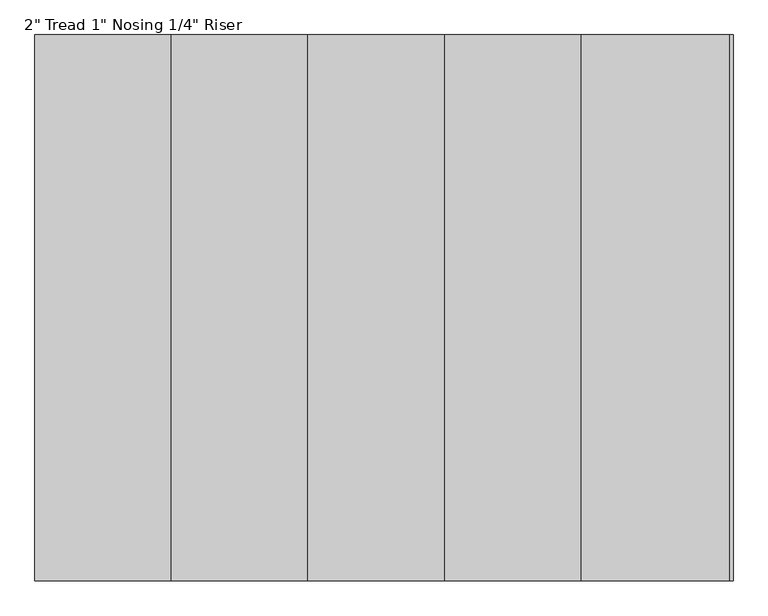
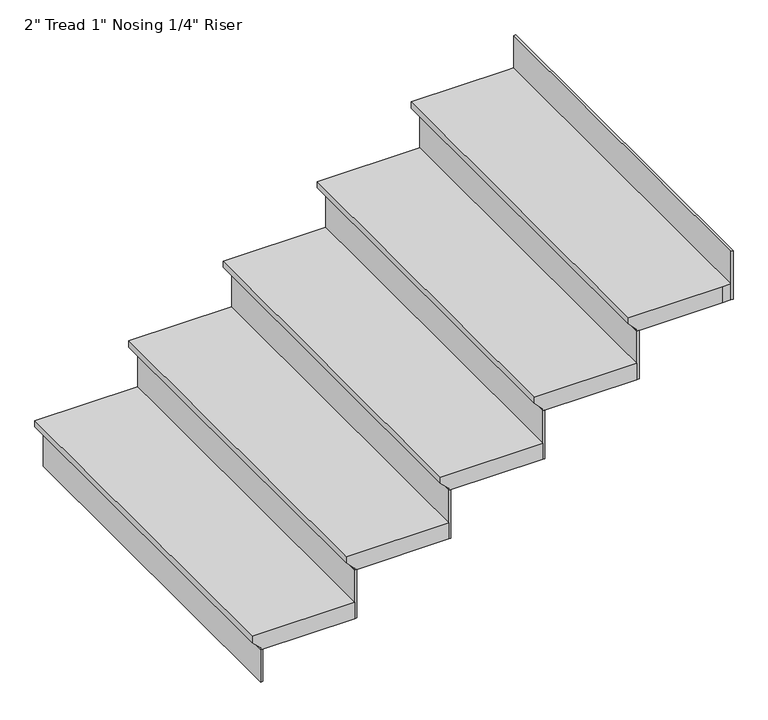
"""IFC4 building model written with IfcOpenShell, lengths in millimetres: stair flight geometry."""

import ifcopenshell
import ifcopenshell.guid

model = None  # the IFC model being written
_history = None  # IfcOwnerHistory: only IFC2X3 demands one
_inside = {}  # id of a spatial element -> (the spatial element, [elements in it])
_under = {}  # id of a project, library or spatial element -> (it, [spatial elements below it])
_declared = {}  # id of a project -> (the project, [libraries it declares])
_typed = {}  # id of a type object -> (the type object, [elements of that type])
_made_of = {}  # id of a material, layer set ... -> (it, [elements and type objects made of it])


def new_model(schema):
    """Start an empty IFC model of exactly this schema.

    Asked for "IFC4X3", IfcOpenShell would pick the latest addendum, in which some entities
    have other attributes; the version numbers below select the first issue.
    IFC2X3 requires an IfcOwnerHistory on every rooted entity: one is made here for all.
    """
    global model, _history
    if schema == "IFC4X3":
        model = ifcopenshell.file(schema_version=(4, 3, 0, 0))
    else:
        model = ifcopenshell.file(schema=schema)
    _inside.clear()
    _under.clear()
    _declared.clear()
    _typed.clear()
    _made_of.clear()
    _history = None
    if model.schema == "IFC2X3":
        org = make("IfcOrganization", Name="unknown")
        user = make(
            "IfcPersonAndOrganization",
            ThePerson=make("IfcPerson", FamilyName="unknown"),
            TheOrganization=org,
        )
        app = make(
            "IfcApplication",
            ApplicationDeveloper=org,
            Version="unknown",
            ApplicationFullName="unknown",
            ApplicationIdentifier="unknown",
        )
        _history = make(
            "IfcOwnerHistory",
            OwningUser=user,
            OwningApplication=app,
            ChangeAction="ADDED",
            CreationDate=0,
        )
    return model


def make(cls, **values):
    """One entity of the class cls with the attributes given. An attribute that is None is left unset."""
    return model.create_entity(
        cls, **{name: value for name, value in values.items() if value is not None}
    )


def rooted(cls, **values):
    """An entity with a GlobalId (a new one), such as an element, a storey or a relation."""
    return make(cls, GlobalId=ifcopenshell.guid.new(), OwnerHistory=_history, **values)


def si_unit(unit_type, name, prefix=None):
    """IfcSIUnit, for example si_unit("LENGTHUNIT", "METRE", prefix="MILLI")."""
    return make("IfcSIUnit", UnitType=unit_type, Prefix=prefix, Name=name)


def assignment(units):
    """IfcUnitAssignment: the units of a project."""
    return None if units is None else make("IfcUnitAssignment", Units=units)


def point(xyz):
    """IfcCartesianPoint."""
    return None if xyz is None else make("IfcCartesianPoint", Coordinates=xyz)


def direction(xyz):
    """IfcDirection."""
    return None if xyz is None else make("IfcDirection", DirectionRatios=xyz)


def frame(location, z_axis=None, x_axis=None):
    """IfcAxis2Placement3D, a coordinate frame: its origin and axes. An axis left out is left unset."""
    return make(
        "IfcAxis2Placement3D",
        Location=point(location),
        Axis=direction(z_axis),
        RefDirection=direction(x_axis),
    )


def origin():
    """The frame at (0, 0, 0) with its axes left unset."""
    return frame((0.0, 0.0, 0.0))


def place(relative_to, where):
    """IfcLocalPlacement: puts the frame where relative to a parent placement (None: the world)."""
    return make(
        "IfcLocalPlacement", PlacementRelTo=relative_to, RelativePlacement=where
    )


def context(
    kind, dimensions, precision=None, world=None, true_north=None, identifier=None
):
    """IfcGeometricRepresentationContext, for example the 3D "Model" context."""
    return make(
        "IfcGeometricRepresentationContext",
        ContextIdentifier=identifier,
        ContextType=kind,
        CoordinateSpaceDimension=dimensions,
        Precision=precision,
        WorldCoordinateSystem=world,
        TrueNorth=true_north,
    )


def project(units=None, contexts=None):
    """IfcProject with its units and contexts."""
    return rooted(
        "IfcProject",
        Name="project",
        RepresentationContexts=contexts,
        UnitsInContext=assignment(units),
    )


def spatial(cls, under=None, at=None, **own):
    """A site, building, storey or space (cls), placed at a placement, below another one or the project."""
    s = rooted(cls, ObjectPlacement=at, **own)
    if under is not None:
        _under.setdefault(under.id(), (under, []))[1].append(s)
    return s


def faces_of(points, faces, orient=None, outer=None):
    """IfcFace entities. A face is a list of loops; a loop is a list of indices into points, from 0.

    orient and outer hold one flag for each loop. By default every Orientation is true, the
    first loop of a face is its IfcFaceOuterBound and the others are IfcFaceBound.
    """
    made = []
    for i, loops in enumerate(faces):
        bounds = []
        for j, loop in enumerate(loops):
            is_outer = j == 0 if outer is None else outer[i][j]
            bounds.append(
                make(
                    "IfcFaceOuterBound" if is_outer else "IfcFaceBound",
                    Bound=make("IfcPolyLoop", Polygon=[points[k] for k in loop]),
                    Orientation=True if orient is None else orient[i][j],
                )
            )
        made.append(make("IfcFace", Bounds=bounds))
    return made


def faceted_brep(points, faces, orient=None, outer=None, voids=None):
    """IfcFacetedBrep: a solid bounded by flat faces; with voids (closed shells), ...WithVoids."""
    shared = [point(p) for p in points]
    hull = make("IfcClosedShell", CfsFaces=faces_of(shared, faces, orient, outer))
    if voids is None:
        return make("IfcFacetedBrep", Outer=hull)
    return make(
        "IfcFacetedBrepWithVoids",
        Outer=hull,
        Voids=[
            make(cls, CfsFaces=faces_of(shared, fs, o, b)) for cls, fs, o, b in voids
        ],
    )


def shape(context_of_items, identifier, shape_type, items):
    """IfcShapeRepresentation: the items that make up one representation, for example the "Body"."""
    return make(
        "IfcShapeRepresentation",
        ContextOfItems=context_of_items,
        RepresentationIdentifier=identifier,
        RepresentationType=shape_type,
        Items=items,
    )


def source(mapping_origin, context_of_items, identifier, shape_type, items):
    """IfcRepresentationMap: a shape defined once, which mapped items show again and again."""
    return make(
        "IfcRepresentationMap",
        MappingOrigin=mapping_origin,
        MappedRepresentation=shape(context_of_items, identifier, shape_type, items),
    )


def transform(
    local_origin,
    x_axis=None,
    y_axis=None,
    z_axis=None,
    scale=None,
    scale2=None,
    scale3=None,
    uniform=True,
):
    """IfcCartesianTransformationOperator3D, or its non-uniform kind. x_axis, y_axis, z_axis: its Axis1, 2, 3."""
    if uniform:
        return make(
            "IfcCartesianTransformationOperator3D",
            Axis1=direction(x_axis),
            Axis2=direction(y_axis),
            LocalOrigin=point(local_origin),
            Scale=scale,
            Axis3=direction(z_axis),
        )
    return make(
        "IfcCartesianTransformationOperator3DnonUniform",
        Axis1=direction(x_axis),
        Axis2=direction(y_axis),
        LocalOrigin=point(local_origin),
        Scale=scale,
        Axis3=direction(z_axis),
        Scale2=scale2,
        Scale3=scale3,
    )


def mapped(mapping_source, mapping_target):
    """IfcMappedItem: shows the shape of a source again, moved by a transform."""
    return make(
        "IfcMappedItem", MappingSource=mapping_source, MappingTarget=mapping_target
    )


def made_of(thing, what):
    """Note that an element or type object is made of a material, layer set ...; save() writes the relation."""
    if what is not None:
        _made_of.setdefault(what.id(), (what, []))[1].append(thing)
    return thing


def element(
    cls,
    number,
    at=None,
    inside=None,
    cuts=None,
    type_object=None,
    material=None,
    context=None,
    identifier="Body",
    shape_type=None,
    held_by="IfcProductDefinitionShape",
    body=None,
    shapes=None,
    **own,
):
    """One element of the class cls, such as IfcWall. Its Tag is "e" and its number.

    at: its placement. inside: the storey or other place that contains it. cuts: it is an
    opening in that element (IfcRelVoidsElement). A single representation is given by context,
    identifier, shape_type and body (its items); several are given by shapes. held_by: the class
    of the entity that holds the representations. save() writes the other relations.
    """
    e = rooted(cls, Tag="e%d" % number, ObjectPlacement=at, **own)
    if body is not None:
        shapes = [shape(context, identifier, shape_type, body)]
    if shapes is not None:
        e.Representation = make(held_by, Representations=shapes)
    if inside is not None:
        _inside.setdefault(inside.id(), (inside, []))[1].append(e)
    if cuts is not None:
        rooted(
            "IfcRelVoidsElement", RelatingBuildingElement=cuts, RelatedOpeningElement=e
        )
    if type_object is not None:
        _typed.setdefault(type_object.id(), (type_object, []))[1].append(e)
    return made_of(e, material)


def aggregate(whole, parts):
    """IfcRelAggregates: a whole, such as a stair, and the parts it consists of."""
    return rooted("IfcRelAggregates", RelatingObject=whole, RelatedObjects=parts)


def save(model, path):
    """Write the relations noted so far, then the file.

    IfcRelAggregates (storeys below a building ...), IfcRelContainedInSpatialStructure (elements
    in a storey), IfcRelDefinesByType, IfcRelAssociatesMaterial and IfcRelDeclares: one each for
    every whole, place, type object, material and project.
    """
    for whole, parts in _under.values():
        aggregate(whole, parts)
    for where, things in _inside.values():
        rooted(
            "IfcRelContainedInSpatialStructure",
            RelatedElements=things,
            RelatingStructure=where,
        )
    for kind, things in _typed.values():
        rooted("IfcRelDefinesByType", RelatedObjects=things, RelatingType=kind)
    for what, things in _made_of.values():
        rooted("IfcRelAssociatesMaterial", RelatedObjects=things, RelatingMaterial=what)
    for by, libraries in _declared.values():
        rooted("IfcRelDeclares", RelatingContext=by, RelatedDefinitions=libraries)
    model.write(path)


def stair_flight_71736acc(model_context):
    return source(origin(), model_context, "Body", "Brep", [
        faceted_brep([(-2715.2122732, 8132.6265304, -781.05), (-2715.2122732, 8132.6265304, -762.0), (-2715.2122732, 9250.2265304, -762.0), (-2715.2122732, 9250.2265304, -781.05), (-2689.8122732, 8132.6265304, -806.45), (-2689.8122732, 9250.2265304, -806.45), (-2410.4122732, 8132.6265304, -762.0), (-2410.4122732, 9250.2265304, -762.0), (-2689.8122732, 9250.2265304, -812.8), (-2410.4122732, 9250.2265304, -812.8), (-2410.4122732, 8132.6265304, -812.8), (-2689.8122732, 8132.6265304, -812.8)], [[[0, 1, 2, 3]], [[4, 0, 3, 5]], [[2, 1, 6, 7]], [[8, 9, 10, 11]], [[2, 7, 9, 8, 5, 3]], [[8, 11, 4, 5]], [[6, 1, 0, 4, 11, 10]], [[7, 6, 10, 9]]]),
        faceted_brep([(-2689.8122732, 8132.6265304, -812.8), (-2689.8122732, 8132.6265304, -914.4), (-2683.4622732, 8132.6265304, -914.4), (-2683.4622732, 8132.6265304, -812.8), (-2689.8122732, 9250.2265304, -812.8), (-2683.4622732, 9250.2265304, -812.8), (-2683.4622732, 9250.2265304, -914.4), (-2689.8122732, 9250.2265304, -914.4)], [[[0, 1, 2, 3]], [[4, 5, 6, 7]], [[1, 0, 4, 7]], [[2, 1, 7, 6]], [[3, 2, 6, 5]], [[0, 3, 5, 4]]]),
        faceted_brep([(-2410.4122732, 8132.6265304, -660.4), (-2410.4122732, 8132.6265304, -812.8), (-2404.0622732, 8132.6265304, -812.8), (-2404.0622732, 8132.6265304, -660.4), (-2410.4122732, 9250.2265304, -660.4), (-2404.0622732, 9250.2265304, -660.4), (-2404.0622732, 9250.2265304, -812.8), (-2410.4122732, 9250.2265304, -812.8)], [[[0, 1, 2, 3]], [[4, 5, 6, 7]], [[1, 0, 4, 7]], [[2, 1, 7, 6]], [[3, 2, 6, 5]], [[0, 3, 5, 4]]]),
        faceted_brep([(-2435.8122732, 9250.2265304, -609.6), (-2435.8122732, 8132.6265304, -609.6), (-2131.0122732, 8132.6265304, -609.6), (-2131.0122732, 9250.2265304, -609.6), (-2410.4122732, 9250.2265304, -660.4), (-2131.0122732, 9250.2265304, -660.4), (-2131.0122732, 8132.6265304, -660.4), (-2410.4122732, 8132.6265304, -660.4), (-2410.4122732, 9250.2265304, -654.05), (-2435.8122732, 9250.2265304, -628.65), (-2410.4122732, 8132.6265304, -654.05), (-2435.8122732, 8132.6265304, -628.65)], [[[0, 1, 2, 3]], [[4, 5, 6, 7]], [[0, 3, 5, 4, 8, 9]], [[4, 7, 10, 8]], [[2, 1, 11, 10, 7, 6]], [[3, 2, 6, 5]], [[11, 1, 0, 9]], [[10, 11, 9, 8]]]),
        faceted_brep([(-2131.0122732, 8132.6265304, -508.0), (-2131.0122732, 8132.6265304, -660.4), (-2124.6622732, 8132.6265304, -660.4), (-2124.6622732, 8132.6265304, -508.0), (-2131.0122732, 9250.2265304, -508.0), (-2124.6622732, 9250.2265304, -508.0), (-2124.6622732, 9250.2265304, -660.4), (-2131.0122732, 9250.2265304, -660.4)], [[[0, 1, 2, 3]], [[4, 5, 6, 7]], [[1, 0, 4, 7]], [[2, 1, 7, 6]], [[3, 2, 6, 5]], [[0, 3, 5, 4]]]),
        faceted_brep([(-2156.4122732, 9250.2265304, -457.2), (-2156.4122732, 8132.6265304, -457.2), (-1851.6122732, 8132.6265304, -457.2), (-1851.6122732, 9250.2265304, -457.2), (-2131.0122732, 9250.2265304, -508.0), (-1851.6122732, 9250.2265304, -508.0), (-1851.6122732, 8132.6265304, -508.0), (-2131.0122732, 8132.6265304, -508.0), (-2131.0122732, 9250.2265304, -501.65), (-2156.4122732, 9250.2265304, -476.25), (-2131.0122732, 8132.6265304, -501.65), (-2156.4122732, 8132.6265304, -476.25)], [[[0, 1, 2, 3]], [[4, 5, 6, 7]], [[0, 3, 5, 4, 8, 9]], [[4, 7, 10, 8]], [[2, 1, 11, 10, 7, 6]], [[3, 2, 6, 5]], [[11, 1, 0, 9]], [[10, 11, 9, 8]]]),
        faceted_brep([(-1851.6122732, 8132.6265304, -355.6), (-1851.6122732, 8132.6265304, -508.0), (-1845.2622732, 8132.6265304, -508.0), (-1845.2622732, 8132.6265304, -355.6), (-1851.6122732, 9250.2265304, -355.6), (-1845.2622732, 9250.2265304, -355.6), (-1845.2622732, 9250.2265304, -508.0), (-1851.6122732, 9250.2265304, -508.0)], [[[0, 1, 2, 3]], [[4, 5, 6, 7]], [[1, 0, 4, 7]], [[2, 1, 7, 6]], [[3, 2, 6, 5]], [[0, 3, 5, 4]]]),
        faceted_brep([(-1877.0122732, 9250.2265304, -304.8), (-1877.0122732, 8132.6265304, -304.8), (-1572.2122732, 8132.6265304, -304.8), (-1572.2122732, 9250.2265304, -304.8), (-1851.6122732, 9250.2265304, -355.6), (-1572.2122732, 9250.2265304, -355.6), (-1572.2122732, 8132.6265304, -355.6), (-1851.6122732, 8132.6265304, -355.6), (-1851.6122732, 9250.2265304, -349.25), (-1877.0122732, 9250.2265304, -323.85), (-1851.6122732, 8132.6265304, -349.25), (-1877.0122732, 8132.6265304, -323.85)], [[[0, 1, 2, 3]], [[4, 5, 6, 7]], [[0, 3, 5, 4, 8, 9]], [[4, 7, 10, 8]], [[2, 1, 11, 10, 7, 6]], [[3, 2, 6, 5]], [[11, 1, 0, 9]], [[10, 11, 9, 8]]]),
        faceted_brep([(-1292.8122732, 8132.6265304, -50.8), (-1292.8122732, 8132.6265304, -203.2), (-1286.4622732, 8132.6265304, -203.2), (-1286.4622732, 8132.6265304, -50.8), (-1292.8122732, 9250.2265304, -50.8), (-1286.4622732, 9250.2265304, -50.8), (-1286.4622732, 9250.2265304, -203.2), (-1292.8122732, 9250.2265304, -203.2)], [[[0, 1, 2, 3]], [[4, 5, 6, 7]], [[1, 0, 4, 7]], [[2, 1, 7, 6]], [[3, 2, 6, 5]], [[0, 3, 5, 4]]]),
        faceted_brep([(-1572.2122732, 8132.6265304, -203.2), (-1572.2122732, 8132.6265304, -355.6), (-1565.8622732, 8132.6265304, -355.6), (-1565.8622732, 8132.6265304, -203.2), (-1572.2122732, 9250.2265304, -203.2), (-1565.8622732, 9250.2265304, -203.2), (-1565.8622732, 9250.2265304, -355.6), (-1572.2122732, 9250.2265304, -355.6)], [[[0, 1, 2, 3]], [[4, 5, 6, 7]], [[1, 0, 4, 7]], [[2, 1, 7, 6]], [[3, 2, 6, 5]], [[0, 3, 5, 4]]]),
        faceted_brep([(-1292.8122732, 9250.2265304, -152.4), (-1318.2122732, 9250.2265304, -152.4), (-1597.6122732, 9250.2265304, -152.4), (-1597.6122732, 8132.6265304, -152.4), (-1318.2122732, 8132.6265304, -152.4), (-1292.8122732, 8132.6265304, -152.4), (-1318.2122732, 9250.2265304, -203.2), (-1292.8122732, 9250.2265304, -203.2), (-1292.8122732, 8132.6265304, -203.2), (-1318.2122732, 8132.6265304, -203.2), (-1572.2122732, 8132.6265304, -203.2), (-1572.2122732, 9250.2265304, -203.2), (-1572.2122732, 9250.2265304, -196.85), (-1597.6122732, 9250.2265304, -171.45), (-1572.2122732, 8132.6265304, -196.85), (-1597.6122732, 8132.6265304, -171.45)], [[[0, 1, 2, 3, 4, 5]], [[6, 7, 8, 9, 10, 11]], [[1, 0, 7, 6]], [[2, 1, 6, 11, 12, 13]], [[11, 10, 14, 12]], [[4, 3, 15, 14, 10, 9]], [[5, 4, 9, 8]], [[0, 5, 8, 7]], [[15, 3, 2, 13]], [[14, 15, 13, 12]]]),
    ])


if __name__ == "__main__":
    model = new_model("IFC4")
    model_context = context("Model", 3, world=origin())
    ifc_project = project(units=[si_unit("LENGTHUNIT", "METRE", prefix="MILLI")], contexts=[model_context])
    site = spatial("IfcSite", under=ifc_project)
    building = spatial("IfcBuilding", under=site)
    placement = place(None, origin())
    stair_flight_shape = stair_flight_71736acc(model_context)
    element("IfcStairFlight", 1, ObjectType="2\" Tread 1\" Nosing 1/4\" Riser", at=placement, inside=building, context=model_context, shape_type="MappedRepresentation", body=[
        mapped(stair_flight_shape, transform((0.0, 0.0, 0.0), x_axis=(1.0, 0.0, 0.0), y_axis=(0.0, 1.0, 0.0), z_axis=(0.0, 0.0, 1.0))),
    ])
    save(model, "model.ifc")
